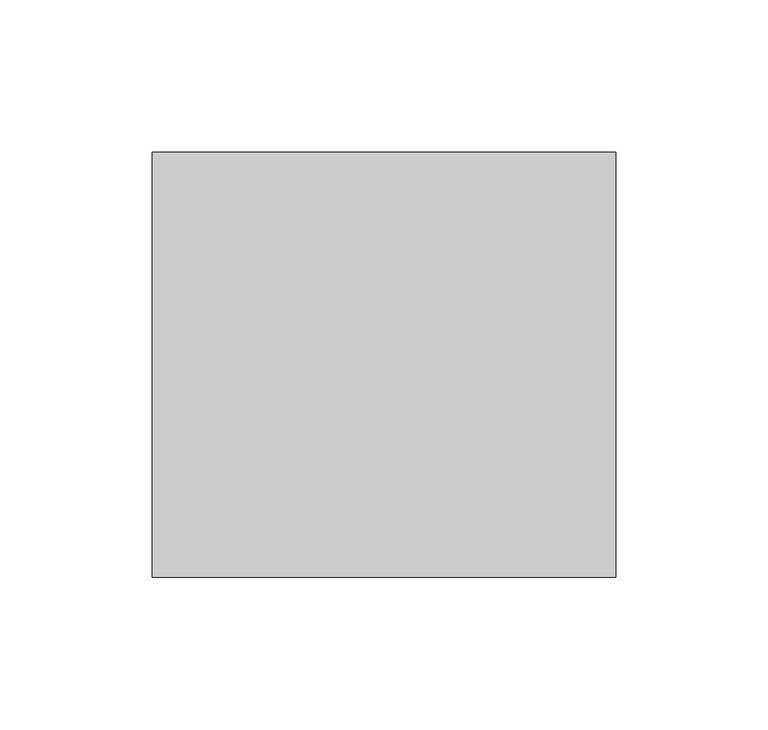
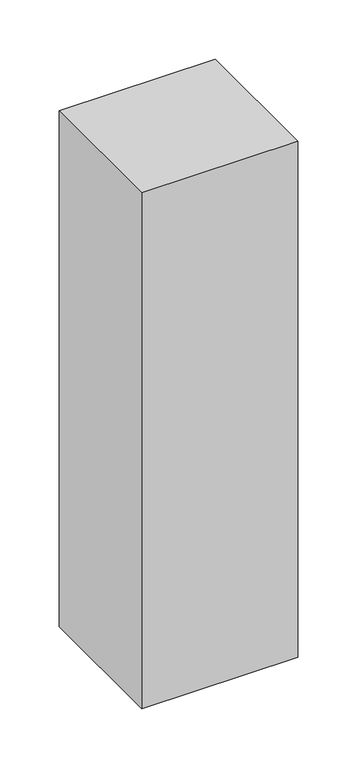
"""IFC4 building model written with IfcOpenShell, lengths in millimetres: proxy geometry, Framing001 475 : Framing001 475."""

import ifcopenshell
import ifcopenshell.guid

model = None  # the IFC model being written
_history = None  # IfcOwnerHistory: only IFC2X3 demands one
_inside = {}  # id of a spatial element -> (the spatial element, [elements in it])
_under = {}  # id of a project, library or spatial element -> (it, [spatial elements below it])
_declared = {}  # id of a project -> (the project, [libraries it declares])
_typed = {}  # id of a type object -> (the type object, [elements of that type])
_made_of = {}  # id of a material, layer set ... -> (it, [elements and type objects made of it])


def new_model(schema):
    """Start an empty IFC model of exactly this schema.

    Asked for "IFC4X3", IfcOpenShell would pick the latest addendum, in which some entities
    have other attributes; the version numbers below select the first issue.
    IFC2X3 requires an IfcOwnerHistory on every rooted entity: one is made here for all.
    """
    global model, _history
    if schema == "IFC4X3":
        model = ifcopenshell.file(schema_version=(4, 3, 0, 0))
    else:
        model = ifcopenshell.file(schema=schema)
    _inside.clear()
    _under.clear()
    _declared.clear()
    _typed.clear()
    _made_of.clear()
    _history = None
    if model.schema == "IFC2X3":
        org = make("IfcOrganization", Name="unknown")
        user = make(
            "IfcPersonAndOrganization",
            ThePerson=make("IfcPerson", FamilyName="unknown"),
            TheOrganization=org,
        )
        app = make(
            "IfcApplication",
            ApplicationDeveloper=org,
            Version="unknown",
            ApplicationFullName="unknown",
            ApplicationIdentifier="unknown",
        )
        _history = make(
            "IfcOwnerHistory",
            OwningUser=user,
            OwningApplication=app,
            ChangeAction="ADDED",
            CreationDate=0,
        )
    return model


def make(cls, **values):
    """One entity of the class cls with the attributes given. An attribute that is None is left unset."""
    return model.create_entity(
        cls, **{name: value for name, value in values.items() if value is not None}
    )


def rooted(cls, **values):
    """An entity with a GlobalId (a new one), such as an element, a storey or a relation."""
    return make(cls, GlobalId=ifcopenshell.guid.new(), OwnerHistory=_history, **values)


def si_unit(unit_type, name, prefix=None):
    """IfcSIUnit, for example si_unit("LENGTHUNIT", "METRE", prefix="MILLI")."""
    return make("IfcSIUnit", UnitType=unit_type, Prefix=prefix, Name=name)


def assignment(units):
    """IfcUnitAssignment: the units of a project."""
    return None if units is None else make("IfcUnitAssignment", Units=units)


def point(xyz):
    """IfcCartesianPoint."""
    return None if xyz is None else make("IfcCartesianPoint", Coordinates=xyz)


def direction(xyz):
    """IfcDirection."""
    return None if xyz is None else make("IfcDirection", DirectionRatios=xyz)


def frame(location, z_axis=None, x_axis=None):
    """IfcAxis2Placement3D, a coordinate frame: its origin and axes. An axis left out is left unset."""
    return make(
        "IfcAxis2Placement3D",
        Location=point(location),
        Axis=direction(z_axis),
        RefDirection=direction(x_axis),
    )


def origin():
    """The frame at (0, 0, 0) with its axes left unset."""
    return frame((0.0, 0.0, 0.0))


def place(relative_to, where):
    """IfcLocalPlacement: puts the frame where relative to a parent placement (None: the world)."""
    return make(
        "IfcLocalPlacement", PlacementRelTo=relative_to, RelativePlacement=where
    )


def context(
    kind, dimensions, precision=None, world=None, true_north=None, identifier=None
):
    """IfcGeometricRepresentationContext, for example the 3D "Model" context."""
    return make(
        "IfcGeometricRepresentationContext",
        ContextIdentifier=identifier,
        ContextType=kind,
        CoordinateSpaceDimension=dimensions,
        Precision=precision,
        WorldCoordinateSystem=world,
        TrueNorth=true_north,
    )


def project(units=None, contexts=None):
    """IfcProject with its units and contexts."""
    return rooted(
        "IfcProject",
        Name="project",
        RepresentationContexts=contexts,
        UnitsInContext=assignment(units),
    )


def spatial(cls, under=None, at=None, **own):
    """A site, building, storey or space (cls), placed at a placement, below another one or the project."""
    s = rooted(cls, ObjectPlacement=at, **own)
    if under is not None:
        _under.setdefault(under.id(), (under, []))[1].append(s)
    return s


def polyline(points):
    """IfcPolyline through the points."""
    return make("IfcPolyline", Points=[point(p) for p in points])


def outline(outer, holes=None, kind="AREA"):
    """IfcArbitraryClosedProfileDef: a profile drawn as a closed curve; with holes, ...WithVoids."""
    if holes is None:
        return make("IfcArbitraryClosedProfileDef", ProfileType=kind, OuterCurve=outer)
    return make(
        "IfcArbitraryProfileDefWithVoids",
        ProfileType=kind,
        OuterCurve=outer,
        InnerCurves=holes,
    )


def extrude(swept, where, along, depth):
    """IfcExtrudedAreaSolid: the profile swept, set in the frame where, extruded along a direction by depth."""
    return make(
        "IfcExtrudedAreaSolid",
        SweptArea=swept,
        Position=where,
        ExtrudedDirection=direction(along),
        Depth=depth,
    )


def shape(context_of_items, identifier, shape_type, items):
    """IfcShapeRepresentation: the items that make up one representation, for example the "Body"."""
    return make(
        "IfcShapeRepresentation",
        ContextOfItems=context_of_items,
        RepresentationIdentifier=identifier,
        RepresentationType=shape_type,
        Items=items,
    )


def source(mapping_origin, context_of_items, identifier, shape_type, items):
    """IfcRepresentationMap: a shape defined once, which mapped items show again and again."""
    return make(
        "IfcRepresentationMap",
        MappingOrigin=mapping_origin,
        MappedRepresentation=shape(context_of_items, identifier, shape_type, items),
    )


def transform(
    local_origin,
    x_axis=None,
    y_axis=None,
    z_axis=None,
    scale=None,
    scale2=None,
    scale3=None,
    uniform=True,
):
    """IfcCartesianTransformationOperator3D, or its non-uniform kind. x_axis, y_axis, z_axis: its Axis1, 2, 3."""
    if uniform:
        return make(
            "IfcCartesianTransformationOperator3D",
            Axis1=direction(x_axis),
            Axis2=direction(y_axis),
            LocalOrigin=point(local_origin),
            Scale=scale,
            Axis3=direction(z_axis),
        )
    return make(
        "IfcCartesianTransformationOperator3DnonUniform",
        Axis1=direction(x_axis),
        Axis2=direction(y_axis),
        LocalOrigin=point(local_origin),
        Scale=scale,
        Axis3=direction(z_axis),
        Scale2=scale2,
        Scale3=scale3,
    )


def mapped(mapping_source, mapping_target):
    """IfcMappedItem: shows the shape of a source again, moved by a transform."""
    return make(
        "IfcMappedItem", MappingSource=mapping_source, MappingTarget=mapping_target
    )


def made_of(thing, what):
    """Note that an element or type object is made of a material, layer set ...; save() writes the relation."""
    if what is not None:
        _made_of.setdefault(what.id(), (what, []))[1].append(thing)
    return thing


def element(
    cls,
    number,
    at=None,
    inside=None,
    cuts=None,
    type_object=None,
    material=None,
    context=None,
    identifier="Body",
    shape_type=None,
    held_by="IfcProductDefinitionShape",
    body=None,
    shapes=None,
    **own,
):
    """One element of the class cls, such as IfcWall. Its Tag is "e" and its number.

    at: its placement. inside: the storey or other place that contains it. cuts: it is an
    opening in that element (IfcRelVoidsElement). A single representation is given by context,
    identifier, shape_type and body (its items); several are given by shapes. held_by: the class
    of the entity that holds the representations. save() writes the other relations.
    """
    e = rooted(cls, Tag="e%d" % number, ObjectPlacement=at, **own)
    if body is not None:
        shapes = [shape(context, identifier, shape_type, body)]
    if shapes is not None:
        e.Representation = make(held_by, Representations=shapes)
    if inside is not None:
        _inside.setdefault(inside.id(), (inside, []))[1].append(e)
    if cuts is not None:
        rooted(
            "IfcRelVoidsElement", RelatingBuildingElement=cuts, RelatedOpeningElement=e
        )
    if type_object is not None:
        _typed.setdefault(type_object.id(), (type_object, []))[1].append(e)
    return made_of(e, material)


def aggregate(whole, parts):
    """IfcRelAggregates: a whole, such as a stair, and the parts it consists of."""
    return rooted("IfcRelAggregates", RelatingObject=whole, RelatedObjects=parts)


def save(model, path):
    """Write the relations noted so far, then the file.

    IfcRelAggregates (storeys below a building ...), IfcRelContainedInSpatialStructure (elements
    in a storey), IfcRelDefinesByType, IfcRelAssociatesMaterial and IfcRelDeclares: one each for
    every whole, place, type object, material and project.
    """
    for whole, parts in _under.values():
        aggregate(whole, parts)
    for where, things in _inside.values():
        rooted(
            "IfcRelContainedInSpatialStructure",
            RelatedElements=things,
            RelatingStructure=where,
        )
    for kind, things in _typed.values():
        rooted("IfcRelDefinesByType", RelatedObjects=things, RelatingType=kind)
    for what, things in _made_of.values():
        rooted("IfcRelAssociatesMaterial", RelatedObjects=things, RelatingMaterial=what)
    for by, libraries in _declared.values():
        rooted("IfcRelDeclares", RelatingContext=by, RelatedDefinitions=libraries)
    model.write(path)


def generic_models_20c3ce23(model_context):
    return source(origin(), model_context, "Body", "SweptSolid", [
        extrude(outline(polyline([(4322.6883192, 10278.0250834), (4322.6883192, 10417.7250834), (4475.0883192, 10417.7250834), (4475.0883192, 10278.0250834), (4322.6883192, 10278.0250834)])), frame((0.0, 0.0, 40138.0976562), z_axis=(0.0, 0.0, 1.0), x_axis=(1.0, 0.0, 0.0)), (0.0, 0.0, 1.0), 533.4),
    ])


if __name__ == "__main__":
    model = new_model("IFC4")
    model_context = context("Model", 3, world=origin())
    ifc_project = project(units=[si_unit("LENGTHUNIT", "METRE", prefix="MILLI")], contexts=[model_context])
    site = spatial("IfcSite", under=ifc_project)
    building = spatial("IfcBuilding", under=site)
    placement = place(None, origin())
    generic_models_shape = generic_models_20c3ce23(model_context)
    element("IfcBuildingElementProxy", 1, Name="Framing001 475 : Framing001 475", ObjectType="Framing001 475 : Framing001 475", at=placement, inside=building, context=model_context, shape_type="MappedRepresentation", body=[
        mapped(generic_models_shape, transform((0.0, 0.0, 0.0), x_axis=(1.0, 0.0, 0.0), y_axis=(0.0, 1.0, 0.0), z_axis=(0.0, 0.0, 1.0))),
    ])
    save(model, "model.ifc")

# Revit data of these elements
# Type "Framing001 475 : Framing001 475"
#   NameOverride = "Framing001"
# Element 1 (IfcBuildingElementProxy, "Framing001 475 : Framing001 475")
#   Materials on its faces: "WOOD FRAMING (SEE STRUCT DWGS)"
# Materials
#   "WOOD FRAMING (SEE STRUCT DWGS)": class "Unassigned", colour RGB 224 188 168, transparency 0, Cost = 0
